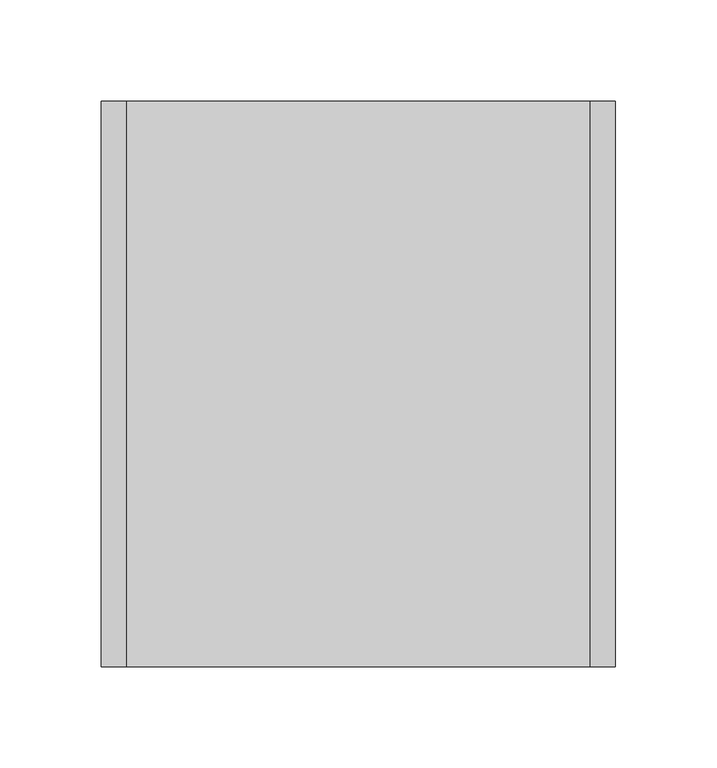
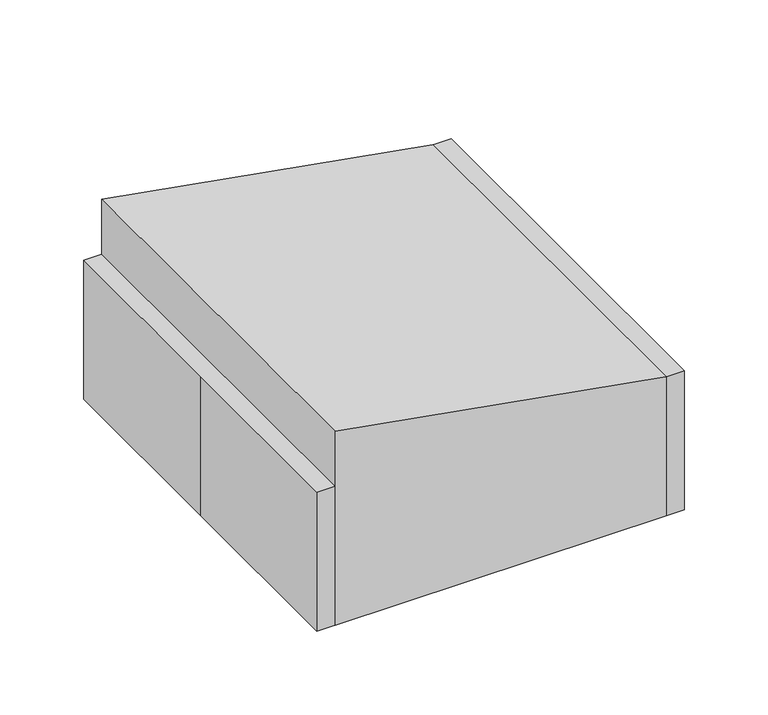
"""IFC4 building model written with IfcOpenShell, lengths in millimetres: proxy geometry, M7660 - Defibrillator-Monitor-Recorder, Portable : M7660 - Defibrillator-Monitor-Recorder, Portable."""

import ifcopenshell
import ifcopenshell.guid

model = None  # the IFC model being written
_history = None  # IfcOwnerHistory: only IFC2X3 demands one
_inside = {}  # id of a spatial element -> (the spatial element, [elements in it])
_under = {}  # id of a project, library or spatial element -> (it, [spatial elements below it])
_declared = {}  # id of a project -> (the project, [libraries it declares])
_typed = {}  # id of a type object -> (the type object, [elements of that type])
_made_of = {}  # id of a material, layer set ... -> (it, [elements and type objects made of it])


def new_model(schema):
    """Start an empty IFC model of exactly this schema.

    Asked for "IFC4X3", IfcOpenShell would pick the latest addendum, in which some entities
    have other attributes; the version numbers below select the first issue.
    IFC2X3 requires an IfcOwnerHistory on every rooted entity: one is made here for all.
    """
    global model, _history
    if schema == "IFC4X3":
        model = ifcopenshell.file(schema_version=(4, 3, 0, 0))
    else:
        model = ifcopenshell.file(schema=schema)
    _inside.clear()
    _under.clear()
    _declared.clear()
    _typed.clear()
    _made_of.clear()
    _history = None
    if model.schema == "IFC2X3":
        org = make("IfcOrganization", Name="unknown")
        user = make(
            "IfcPersonAndOrganization",
            ThePerson=make("IfcPerson", FamilyName="unknown"),
            TheOrganization=org,
        )
        app = make(
            "IfcApplication",
            ApplicationDeveloper=org,
            Version="unknown",
            ApplicationFullName="unknown",
            ApplicationIdentifier="unknown",
        )
        _history = make(
            "IfcOwnerHistory",
            OwningUser=user,
            OwningApplication=app,
            ChangeAction="ADDED",
            CreationDate=0,
        )
    return model


def make(cls, **values):
    """One entity of the class cls with the attributes given. An attribute that is None is left unset."""
    return model.create_entity(
        cls, **{name: value for name, value in values.items() if value is not None}
    )


def rooted(cls, **values):
    """An entity with a GlobalId (a new one), such as an element, a storey or a relation."""
    return make(cls, GlobalId=ifcopenshell.guid.new(), OwnerHistory=_history, **values)


def si_unit(unit_type, name, prefix=None):
    """IfcSIUnit, for example si_unit("LENGTHUNIT", "METRE", prefix="MILLI")."""
    return make("IfcSIUnit", UnitType=unit_type, Prefix=prefix, Name=name)


def assignment(units):
    """IfcUnitAssignment: the units of a project."""
    return None if units is None else make("IfcUnitAssignment", Units=units)


def point(xyz):
    """IfcCartesianPoint."""
    return None if xyz is None else make("IfcCartesianPoint", Coordinates=xyz)


def direction(xyz):
    """IfcDirection."""
    return None if xyz is None else make("IfcDirection", DirectionRatios=xyz)


def frame(location, z_axis=None, x_axis=None):
    """IfcAxis2Placement3D, a coordinate frame: its origin and axes. An axis left out is left unset."""
    return make(
        "IfcAxis2Placement3D",
        Location=point(location),
        Axis=direction(z_axis),
        RefDirection=direction(x_axis),
    )


def origin():
    """The frame at (0, 0, 0) with its axes left unset."""
    return frame((0.0, 0.0, 0.0))


def origin_with_axes():
    """The frame at (0, 0, 0) with the z axis (0, 0, 1) and the x axis (1, 0, 0) written out."""
    return frame((0.0, 0.0, 0.0), z_axis=(0.0, 0.0, 1.0), x_axis=(1.0, 0.0, 0.0))


def place(relative_to, where):
    """IfcLocalPlacement: puts the frame where relative to a parent placement (None: the world)."""
    return make(
        "IfcLocalPlacement", PlacementRelTo=relative_to, RelativePlacement=where
    )


def context(
    kind, dimensions, precision=None, world=None, true_north=None, identifier=None
):
    """IfcGeometricRepresentationContext, for example the 3D "Model" context."""
    return make(
        "IfcGeometricRepresentationContext",
        ContextIdentifier=identifier,
        ContextType=kind,
        CoordinateSpaceDimension=dimensions,
        Precision=precision,
        WorldCoordinateSystem=world,
        TrueNorth=true_north,
    )


def project(units=None, contexts=None):
    """IfcProject with its units and contexts."""
    return rooted(
        "IfcProject",
        Name="project",
        RepresentationContexts=contexts,
        UnitsInContext=assignment(units),
    )


def spatial(cls, under=None, at=None, **own):
    """A site, building, storey or space (cls), placed at a placement, below another one or the project."""
    s = rooted(cls, ObjectPlacement=at, **own)
    if under is not None:
        _under.setdefault(under.id(), (under, []))[1].append(s)
    return s


def polyline(points):
    """IfcPolyline through the points."""
    return make("IfcPolyline", Points=[point(p) for p in points])


def outline(outer, holes=None, kind="AREA"):
    """IfcArbitraryClosedProfileDef: a profile drawn as a closed curve; with holes, ...WithVoids."""
    if holes is None:
        return make("IfcArbitraryClosedProfileDef", ProfileType=kind, OuterCurve=outer)
    return make(
        "IfcArbitraryProfileDefWithVoids",
        ProfileType=kind,
        OuterCurve=outer,
        InnerCurves=holes,
    )


def extrude(swept, where, along, depth):
    """IfcExtrudedAreaSolid: the profile swept, set in the frame where, extruded along a direction by depth."""
    return make(
        "IfcExtrudedAreaSolid",
        SweptArea=swept,
        Position=where,
        ExtrudedDirection=direction(along),
        Depth=depth,
    )


def shape(context_of_items, identifier, shape_type, items):
    """IfcShapeRepresentation: the items that make up one representation, for example the "Body"."""
    return make(
        "IfcShapeRepresentation",
        ContextOfItems=context_of_items,
        RepresentationIdentifier=identifier,
        RepresentationType=shape_type,
        Items=items,
    )


def source(mapping_origin, context_of_items, identifier, shape_type, items):
    """IfcRepresentationMap: a shape defined once, which mapped items show again and again."""
    return make(
        "IfcRepresentationMap",
        MappingOrigin=mapping_origin,
        MappedRepresentation=shape(context_of_items, identifier, shape_type, items),
    )


def transform(
    local_origin,
    x_axis=None,
    y_axis=None,
    z_axis=None,
    scale=None,
    scale2=None,
    scale3=None,
    uniform=True,
):
    """IfcCartesianTransformationOperator3D, or its non-uniform kind. x_axis, y_axis, z_axis: its Axis1, 2, 3."""
    if uniform:
        return make(
            "IfcCartesianTransformationOperator3D",
            Axis1=direction(x_axis),
            Axis2=direction(y_axis),
            LocalOrigin=point(local_origin),
            Scale=scale,
            Axis3=direction(z_axis),
        )
    return make(
        "IfcCartesianTransformationOperator3DnonUniform",
        Axis1=direction(x_axis),
        Axis2=direction(y_axis),
        LocalOrigin=point(local_origin),
        Scale=scale,
        Axis3=direction(z_axis),
        Scale2=scale2,
        Scale3=scale3,
    )


def mapped(mapping_source, mapping_target):
    """IfcMappedItem: shows the shape of a source again, moved by a transform."""
    return make(
        "IfcMappedItem", MappingSource=mapping_source, MappingTarget=mapping_target
    )


def made_of(thing, what):
    """Note that an element or type object is made of a material, layer set ...; save() writes the relation."""
    if what is not None:
        _made_of.setdefault(what.id(), (what, []))[1].append(thing)
    return thing


def element(
    cls,
    number,
    at=None,
    inside=None,
    cuts=None,
    type_object=None,
    material=None,
    context=None,
    identifier="Body",
    shape_type=None,
    held_by="IfcProductDefinitionShape",
    body=None,
    shapes=None,
    **own,
):
    """One element of the class cls, such as IfcWall. Its Tag is "e" and its number.

    at: its placement. inside: the storey or other place that contains it. cuts: it is an
    opening in that element (IfcRelVoidsElement). A single representation is given by context,
    identifier, shape_type and body (its items); several are given by shapes. held_by: the class
    of the entity that holds the representations. save() writes the other relations.
    """
    e = rooted(cls, Tag="e%d" % number, ObjectPlacement=at, **own)
    if body is not None:
        shapes = [shape(context, identifier, shape_type, body)]
    if shapes is not None:
        e.Representation = make(held_by, Representations=shapes)
    if inside is not None:
        _inside.setdefault(inside.id(), (inside, []))[1].append(e)
    if cuts is not None:
        rooted(
            "IfcRelVoidsElement", RelatingBuildingElement=cuts, RelatedOpeningElement=e
        )
    if type_object is not None:
        _typed.setdefault(type_object.id(), (type_object, []))[1].append(e)
    return made_of(e, material)


def aggregate(whole, parts):
    """IfcRelAggregates: a whole, such as a stair, and the parts it consists of."""
    return rooted("IfcRelAggregates", RelatingObject=whole, RelatedObjects=parts)


def save(model, path):
    """Write the relations noted so far, then the file.

    IfcRelAggregates (storeys below a building ...), IfcRelContainedInSpatialStructure (elements
    in a storey), IfcRelDefinesByType, IfcRelAssociatesMaterial and IfcRelDeclares: one each for
    every whole, place, type object, material and project.
    """
    for whole, parts in _under.values():
        aggregate(whole, parts)
    for where, things in _inside.values():
        rooted(
            "IfcRelContainedInSpatialStructure",
            RelatedElements=things,
            RelatingStructure=where,
        )
    for kind, things in _typed.values():
        rooted("IfcRelDefinesByType", RelatedObjects=things, RelatingType=kind)
    for what, things in _made_of.values():
        rooted("IfcRelAssociatesMaterial", RelatedObjects=things, RelatingMaterial=what)
    for by, libraries in _declared.values():
        rooted("IfcRelDeclares", RelatingContext=by, RelatedDefinitions=libraries)
    model.write(path)


def specialty_equipment_730b47bf(model_context):
    return source(origin(), model_context, "Body", "SweptSolid", [
        extrude(outline(polyline([(101.6, 114.3), (141.9083478, -114.3), (0.0, -114.3), (0.0, 114.3), (101.6, 114.3)])), frame((0.0, -139.7, 0.0), z_axis=(0.0, 1.0, 0.0), x_axis=(0.0, 0.0, 1.0)), (0.0, 0.0, 1.0), 279.4),
        extrude(outline(polyline([(-127.0, 139.7), (127.0, 139.7), (127.0, -139.7), (-127.0, -139.7), (-127.0, 0.0), (-127.0, 139.7)])), origin_with_axes(), (0.0, 0.0, 1.0), 101.6),
    ])


if __name__ == "__main__":
    model = new_model("IFC4")
    model_context = context("Model", 3, world=origin())
    ifc_project = project(units=[si_unit("LENGTHUNIT", "METRE", prefix="MILLI")], contexts=[model_context])
    site = spatial("IfcSite", under=ifc_project)
    building = spatial("IfcBuilding", under=site)
    placement = place(None, origin())
    specialty_equipment_shape = specialty_equipment_730b47bf(model_context)
    element("IfcBuildingElementProxy", 1, Name="M7660 - Defibrillator-Monitor-Recorder, Portable : M7660 - Defibrillator-Monitor-Recorder, Portable", ObjectType="M7660 - Defibrillator-Monitor-Recorder, Portable : M7660 - Defibrillator-Monitor-Recorder, Portable", at=placement, inside=building, context=model_context, shape_type="MappedRepresentation", body=[
        mapped(specialty_equipment_shape, transform((0.0, 0.0, 0.0), x_axis=(1.0, 0.0, 0.0), y_axis=(0.0, 1.0, 0.0), z_axis=(0.0, 0.0, 1.0))),
    ])
    save(model, "model.ifc")

# Revit data of these elements
# Type "M7660 - Defibrillator-Monitor-Recorder, Portable : M7660 - Defibrillator-Monitor-Recorder, Portable"
#   Watts2 = "0"
#   Watts1 = "240"
#   Unit_Issue = "EA"
#   UTIL_6_Misc = "-"
#   UTIL_5_NonMedGas = "-"
#   UTIL_4_MiscGas = "-"
#   UTIL_3_MedGas = "-"
#   UTIL_2_Elec = "A"
#   UTIL_1_WaterDrain = "-"
#   Nomenclature = "Defibrillator/Monitor/Recorder, Portable"
#   NSN = "6530013901460"
#   Location [instance default] = ""
#   JSN = "M7660"
#   Fund_Source_VA = "-"
#   Fund_Source_Navy = "-"
#   Fund_Source_Army = "-"
#   Fund_Source_AF = "-"
#   ELEC_Volts2 = "0"
#   ELEC_Volts1 = "120"
#   ELEC_Phase2 = "0"
#   ELEC_Phase1 = "1"
#   ELEC_HertzSwitch = "0"
#   ELEC_HertzDependent = "0"
#   ELEC_Hertz = "60"
#   ELEC_Amps2 = "0"
#   ELEC_Amps1 = "2"
#   DetailDescription = "Portable defibrillator-monitor-recorder. Integral unit system operable from self-contained rechargeable batteries. ECG may be viewed through paddles or patient cable. Options include external pacing and 12-Lead."
#   CAT_VA = "C"
#   CAT_Navy = "C"
#   CAT_IHS = "-"
#   CAT_Army = "C"
#   CAT_AF = "C"
#   BTUperhour = "0"
#   Weight_IP = 7
#   DIM_Width_IP = 0' - 10"
#   DIM_Height_IP = 0' - 4"
#   DIM_Depth_IP = 0' - 11"
#   finish [instance default] = none
# Element 1 (IfcBuildingElementProxy, "M7660 - Defibrillator-Monitor-Recorder, Portable : M7660 - Defibrillator-Monitor-Recorder, Portable")
#   Location = "TRET3"
#   Materials on its faces: "EquipSpace"
# Materials
#   "EquipSpace": class "Unassigned", colour RGB 221 217 195, transparency 0.5
